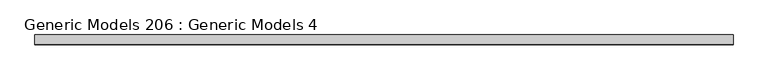
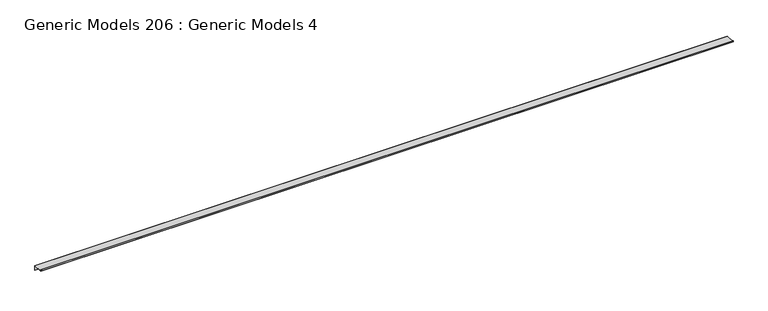
"""IFC4 building model written with IfcOpenShell, lengths in millimetres: proxy geometry, Generic Models 206 : Generic Models 4."""

from ifc_helpers import new_model, si_unit, frame, origin, place, context, project, spatial, polyline, outline, extrude, source, transform, mapped, element, save


def generic_models_206_generic_models_4_6b4eeb48(model_context):
    return source(origin(), model_context, "Body", "SweptSolid", [
        extrude(outline(polyline([(-5469.371169, 126275.2286235), (-5470.164919, 126275.2286235), (-5470.164919, 126364.0018004), (-5646.2681749, 126364.0018004), (-5646.268175, 126390.9335774), (-5645.474425, 126390.9335774), (-5645.4744249, 126364.7955504), (-5469.371169, 126364.7955504), (-5469.371169, 126275.2286235)])), frame((-10234.5171316, 0.0, 0.0), z_axis=(1.0, 0.0, 0.0), x_axis=(0.0, 1.0, 0.0)), (0.0, 0.0, 1.0), 12431.443502),
    ])


if __name__ == "__main__":
    model = new_model("IFC4")
    model_context = context("Model", 3, world=origin())
    ifc_project = project(units=[si_unit("LENGTHUNIT", "METRE", prefix="MILLI")], contexts=[model_context])
    site = spatial("IfcSite", under=ifc_project)
    building = spatial("IfcBuilding", under=site)
    placement = place(None, origin())
    generic_models_206_generic_models_4_shape = generic_models_206_generic_models_4_6b4eeb48(model_context)
    element("IfcBuildingElementProxy", 1, Name="Generic Models 206 : Generic Models 4", ObjectType="Generic Models 206 : Generic Models 4", at=placement, inside=building, context=model_context, shape_type="MappedRepresentation", body=[
        mapped(generic_models_206_generic_models_4_shape, transform((0.0, 0.0, 0.0), x_axis=(1.0, 0.0, 0.0), y_axis=(0.0, 1.0, 0.0), z_axis=(0.0, 0.0, 1.0))),
    ])
    save(model, "model.ifc")

# Revit data of these elements
# Element 1 (IfcBuildingElementProxy, "Generic Models 206 : Generic Models 4")
#   Materials on its faces: "_(2) LAYERS NO. 30 ASTM D226 ASPHALT SATURATED ORGANIC FELT"
# Materials
#   "_(2) LAYERS NO. 30 ASTM D226 ASPHALT SATURATED ORGANIC FELT": class "Generic", colour RGB 67 154 161, transparency 0, Cost = 0
